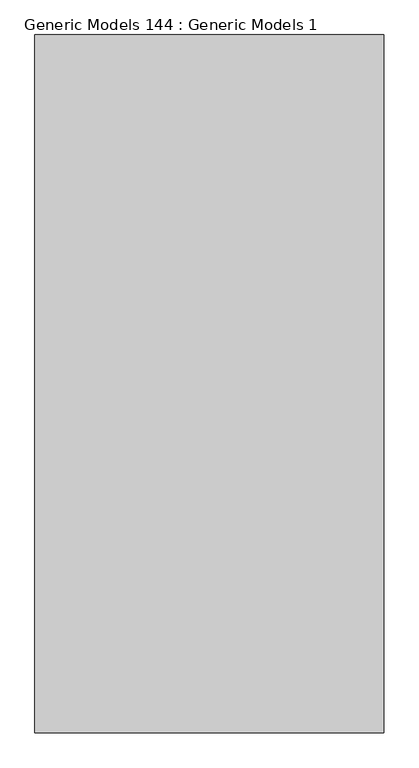
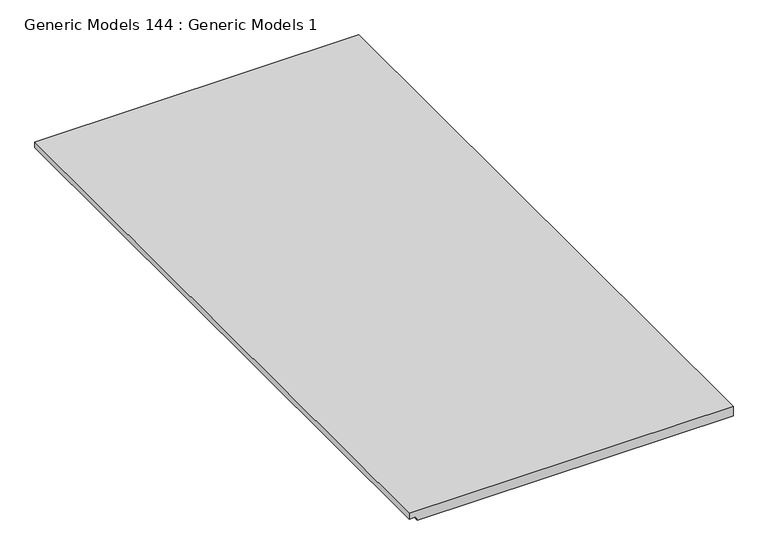
"""IFC4 building model written with IfcOpenShell, lengths in millimetres: proxy geometry, Generic Models 144 : Generic Models 1."""

from ifc_helpers import new_model, si_unit, frame, origin, place, context, project, spatial, polyline, outline, extrude, source, transform, mapped, element, save


def generic_models_144_generic_models_1_0ad20a8b(model_context):
    return source(origin(), model_context, "Body", "SweptSolid", [
        extrude(outline(polyline([(2253.330428, 49813.3451407), (2242.217928, 49813.3451407), (2242.217928, 49826.0451407), (2234.280428, 49828.9341545), (2234.280428, 50422.9451407), (2253.330428, 50422.9451407), (2253.330428, 49813.3451407)])), frame((0.0, 0.0, 0.0), z_axis=(0.0, 1.0, 0.0), x_axis=(0.0, 0.0, 1.0)), (0.0, 0.0, 1.0), 1219.2),
    ])


if __name__ == "__main__":
    model = new_model("IFC4")
    model_context = context("Model", 3, world=origin())
    ifc_project = project(units=[si_unit("LENGTHUNIT", "METRE", prefix="MILLI")], contexts=[model_context])
    site = spatial("IfcSite", under=ifc_project)
    building = spatial("IfcBuilding", under=site)
    placement = place(None, origin())
    generic_models_144_generic_models_1_shape = generic_models_144_generic_models_1_0ad20a8b(model_context)
    element("IfcBuildingElementProxy", 1, Name="Generic Models 144 : Generic Models 1", ObjectType="Generic Models 144 : Generic Models 1", at=placement, inside=building, context=model_context, shape_type="MappedRepresentation", body=[
        mapped(generic_models_144_generic_models_1_shape, transform((0.0, 0.0, 0.0), x_axis=(1.0, 0.0, 0.0), y_axis=(0.0, 1.0, 0.0), z_axis=(0.0, 0.0, 1.0))),
    ])
    save(model, "model.ifc")

# Revit data of these elements
# Element 1 (IfcBuildingElementProxy, "Generic Models 144 : Generic Models 1")
#   Materials on its faces: "CEILING AS SCHEDULED"
# Materials
#   "CEILING AS SCHEDULED": class "Generic", colour RGB 255 255 255, transparency 0, Cost = 0
